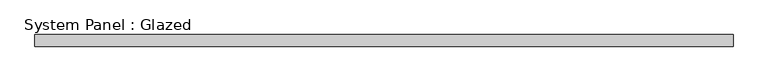
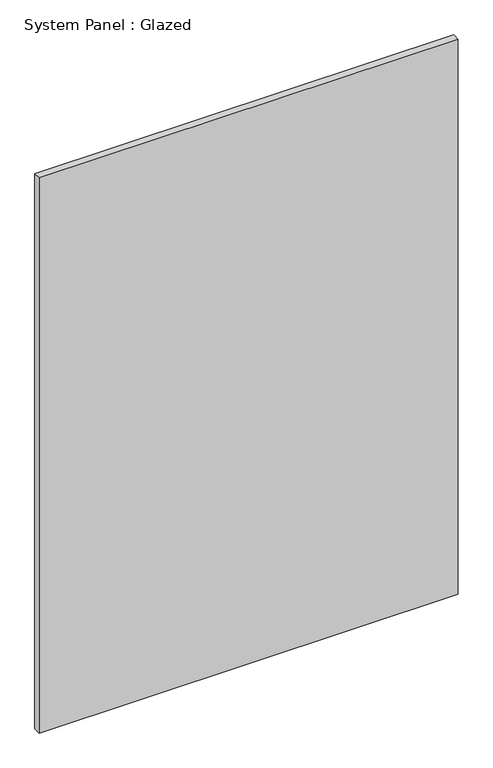
"""IFC4 building model written with IfcOpenShell, lengths in millimetres: plate geometry, System Panel : Glazed."""

from ifc_helpers import new_model, si_unit, origin, origin_with_axes, place, context, project, spatial, polyline, outline, extrude, source, transform, mapped, element, save


def system_panel_glazed_baa26042(model_context):
    return source(origin(), model_context, "Body", "SweptSolid", [
        extrude(outline(polyline([(724.9999999, 24.5), (-724.9999999, 24.5), (-724.9999999, 49.5), (724.9999999, 49.5), (724.9999999, 24.5)])), origin_with_axes(), (0.0, 0.0, 1.0), 2030.4462072),
    ])


if __name__ == "__main__":
    model = new_model("IFC4")
    model_context = context("Model", 3, world=origin())
    ifc_project = project(units=[si_unit("LENGTHUNIT", "METRE", prefix="MILLI")], contexts=[model_context])
    site = spatial("IfcSite", under=ifc_project)
    building = spatial("IfcBuilding", under=site)
    placement = place(None, origin())
    system_panel_glazed_shape = system_panel_glazed_baa26042(model_context)
    element("IfcPlate", 1, ObjectType="System Panel : Glazed", at=placement, inside=building, context=model_context, shape_type="MappedRepresentation", body=[
        mapped(system_panel_glazed_shape, transform((0.0, 0.0, 0.0), x_axis=(1.0, 0.0, 0.0), y_axis=(0.0, 1.0, 0.0), z_axis=(0.0, 0.0, 1.0))),
    ])
    save(model, "model.ifc")

# Revit data of these elements
# Type "System Panel : Glazed"
#   Construction Type Id = "GSP4R"
#   Analytic Construction = "1/8 in Pilkington single glazing"
#   Visual Light Transmittance = 0.9
#   Solar Heat Gain Coefficient = 0.86
#   Heat Transfer Coefficient (U) = 6.7069 W/(m²·K)
#   Define Thermal Properties by = 1
# Element 1 (IfcPlate, "System Panel : Glazed")
#   Materials on its faces: "Glass"
# Materials
#   "Glass": class "Glass", colour RGB 0 128 192, transparency 0.9, Description = "Soda Lime Glass", Cost = 0
